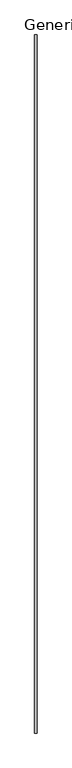
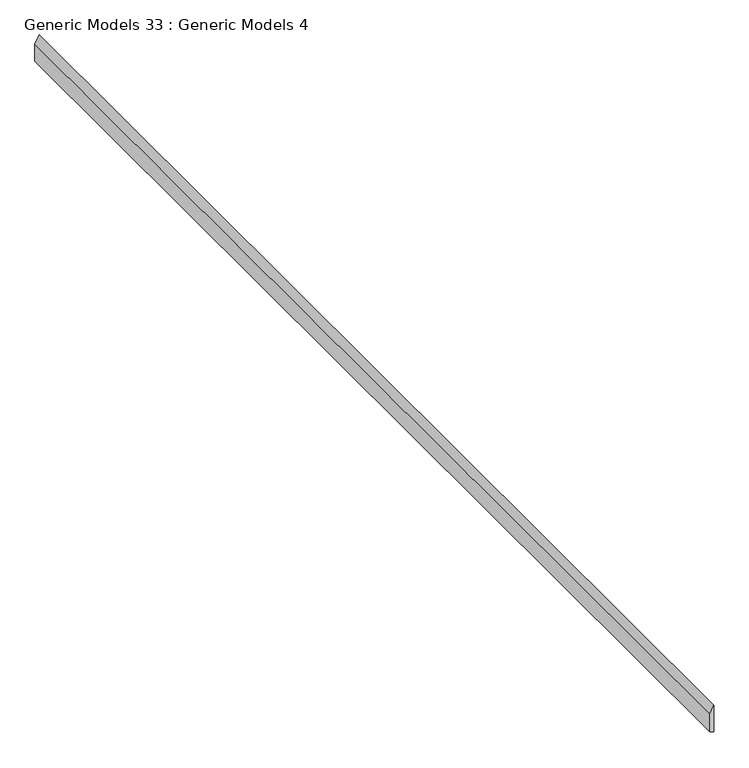
"""IFC4 building model written with IfcOpenShell, lengths in millimetres: proxy geometry, Generic Models 33 : Generic Models 4."""

from ifc_helpers import new_model, si_unit, origin, place, context, project, spatial, faceted_brep, source, transform, mapped, element, save


def generic_models_33_generic_models_4_cbeb7358(model_context):
    return source(origin(), model_context, "Body", "Brep", [
        faceted_brep([(-9250.8536295, 7054.2769662, 126914.4742513), (-9250.8536295, 7054.2769662, 126837.3050625), (-9235.4548796, 7054.2769662, 126832.3554643), (-9233.0736295, 7054.2769662, 126831.5900625), (-9233.0736295, 7054.2769662, 126949.0984618), (-9233.0736295, 11981.8769662, 126949.0984618), (-9233.0736295, 11981.8769662, 126831.5900625), (-9235.4548796, 11981.8769662, 126832.3554643), (-9250.8536295, 11981.8769662, 126837.3050625), (-9250.8536295, 11981.8769662, 126914.4742513)], [[[0, 1, 2, 3, 4]], [[5, 6, 7, 8, 9]], [[1, 0, 9, 8]], [[0, 4, 5, 9]], [[4, 3, 6, 5]], [[1, 8, 7, 6, 3, 2]]]),
    ])


if __name__ == "__main__":
    model = new_model("IFC4")
    model_context = context("Model", 3, world=origin())
    ifc_project = project(units=[si_unit("LENGTHUNIT", "METRE", prefix="MILLI")], contexts=[model_context])
    site = spatial("IfcSite", under=ifc_project)
    building = spatial("IfcBuilding", under=site)
    placement = place(None, origin())
    generic_models_33_generic_models_4_shape = generic_models_33_generic_models_4_cbeb7358(model_context)
    element("IfcBuildingElementProxy", 1, Name="Generic Models 33 : Generic Models 4", ObjectType="Generic Models 33 : Generic Models 4", at=placement, inside=building, context=model_context, shape_type="MappedRepresentation", body=[
        mapped(generic_models_33_generic_models_4_shape, transform((0.0, 0.0, 0.0), x_axis=(1.0, 0.0, 0.0), y_axis=(0.0, 1.0, 0.0), z_axis=(0.0, 0.0, 1.0))),
    ])
    save(model, "model.ifc")

# Revit data of these elements
# Element 1 (IfcBuildingElementProxy, "Generic Models 33 : Generic Models 4")
#   Materials on its faces: "_7/8\" SMOOTH TROWEL EXTERIOR STUCCO (COLOR PER OWNER)"
# Materials
#   "_7/8\" SMOOTH TROWEL EXTERIOR STUCCO (COLOR PER OWNER)": class "Generic", colour RGB 233 233 233, transparency 0, Cost = 0
